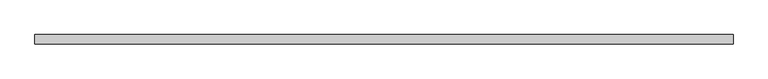
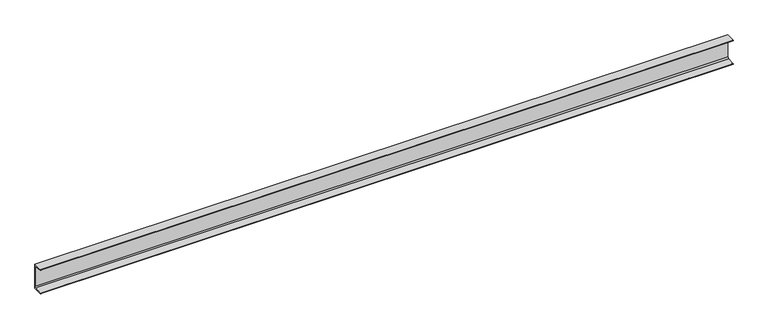
"""IFC4 building model written with IfcOpenShell, lengths in millimetres: beam geometry, C-образный профиль (ГОСТ 8240-89) Балки : [ 22."""

from ifc_helpers import new_model, si_unit, point, frame, frame_2d, origin, place, context, project, spatial, polyline, circle_curve, trimmed, segment, composite_curve, outline, extrude, source, transform, mapped, element, save


def beam_eac20b59(model_context):
    return source(origin(), model_context, "Body", "SweptSolid", [
        extrude(outline(composite_curve([segment(polyline([(22.1, 110.0), (22.1, -110.0), (-59.9, -110.0), (-59.9, -108.9686971)]), True, "CONTINUOUS"), segment(trimmed(circle_curve(frame_2d((-55.9, -108.9686971)), 4.0), [point((-59.9, -108.9686971))], [point((-56.3765809, -104.9971897))], False, "CARTESIAN"), True, "CONTINUOUS"), segment(polyline([(-56.3765809, -104.9971897), (7.8914522, -97.2850257)]), True, "CONTINUOUS"), segment(trimmed(circle_curve(frame_2d((6.7, -87.3562574)), 10.0), [point((7.8914522, -97.2850257))], [point((16.7, -87.3562574))], True, "CARTESIAN"), True, "CONTINUOUS"), segment(polyline([(16.7, -87.3562574), (16.7, 87.3562574)]), True, "CONTINUOUS"), segment(trimmed(circle_curve(frame_2d((6.7, 87.3562574)), 10.0), [point((16.7, 87.3562574))], [point((7.8914522, 97.2850257))], True, "CARTESIAN"), True, "CONTINUOUS"), segment(polyline([(7.8914522, 97.2850257), (-56.3765809, 104.9971897)]), True, "CONTINUOUS"), segment(trimmed(circle_curve(frame_2d((-55.9, 108.9686971)), 4.0), [point((-56.3765809, 104.9971897))], [point((-59.9, 108.9686971))], False, "CARTESIAN"), True, "CONTINUOUS"), segment(polyline([(-59.9, 108.9686971), (-59.9, 110.0), (22.1, 110.0)]), True, "CONTINUOUS")], self_intersect=False)), frame((-2995.0, 0.0, 0.0), z_axis=(1.0, 0.0, 0.0), x_axis=(0.0, 1.0, 0.0)), (0.0, 0.0, 1.0), 5990.0),
    ])


if __name__ == "__main__":
    model = new_model("IFC4")
    model_context = context("Model", 3, world=origin())
    ifc_project = project(units=[si_unit("LENGTHUNIT", "METRE", prefix="MILLI")], contexts=[model_context])
    site = spatial("IfcSite", under=ifc_project)
    building = spatial("IfcBuilding", under=site)
    placement = place(None, origin())
    beam_shape = beam_eac20b59(model_context)
    element("IfcBeam", 1, ObjectType="C-образный профиль (ГОСТ 8240-89) Балки : [ 22", at=placement, inside=building, context=model_context, shape_type="MappedRepresentation", body=[
        mapped(beam_shape, transform((0.0, 0.0, 0.0), x_axis=(1.0, 0.0, 0.0), y_axis=(0.0, 1.0, 0.0), z_axis=(0.0, 0.0, 1.0))),
    ])
    save(model, "model.ifc")

# Revit data of these elements
# Type "C-образный профиль (ГОСТ 8240-89) Балки : [ 22"
#   tf = 9.5 mm
#   ri = 4 mm
#   ra = 10 mm
#   W = 0.20594
#   Vz = 110 mm
#   Vy = 59.9 mm
#   Vpz = 110 mm
#   Vpy = 22.1 mm
#   Уклон = 0.12
#   Length [instance default] = 1500 mm
#   bf = 82 mm
#   d = 220 mm
#   tw = 5.4 mm
#   A = 0.00267 m²
#   Structural Material [instance default] = Металл - Сталь - 345 МПa
#   Assembly Code = ""
# Element 1 (IfcBeam, "C-образный профиль (ГОСТ 8240-89) Балки : [ 22")
#   Structural Material = C235
#   Materials on its faces: "C235"
# Materials
#   "Металл - Сталь - 345 МПa": class "Металл", colour RGB 247 247 247, transparency 0
#   "C235": class "Не назначено", colour RGB 0 0 0, transparency 0
